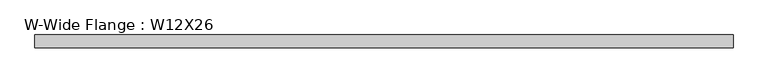
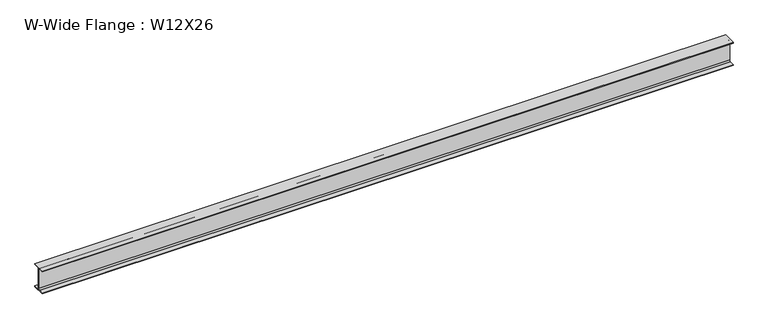
"""IFC4 building model written with IfcOpenShell, lengths in millimetres: beam geometry, W-Wide Flange : W12X26."""

from ifc_helpers import new_model, si_unit, point, frame, frame_2d, origin, place, context, project, spatial, polyline, circle_curve, trimmed, segment, composite_curve, outline, extrude, source, transform, mapped, element, save


def w_wide_flange_w12x26_21dbd052(model_context):
    return source(origin(), model_context, "Body", "SweptSolid", [
        extrude(outline(composite_curve([segment(polyline([(82.4011719, -145.5539063), (82.4011719, -155.178125), (-82.4011719, -155.178125), (-82.4011719, -145.5539063), (-20.2902344, -145.5539063)]), True, "CONTINUOUS"), segment(trimmed(circle_curve(frame_2d((-20.2902344, -128.190625)), 17.3632812), [point((-20.2902344, -145.5539063))], [point((-2.9269531, -128.190625))], True, "CARTESIAN"), True, "CONTINUOUS"), segment(polyline([(-2.9269531, -128.190625), (-2.9269531, 128.190625)]), True, "CONTINUOUS"), segment(trimmed(circle_curve(frame_2d((-20.2902344, 128.190625)), 17.3632812), [point((-2.9269531, 128.190625))], [point((-20.2902344, 145.5539062))], True, "CARTESIAN"), True, "CONTINUOUS"), segment(polyline([(-20.2902344, 145.5539062), (-82.4011719, 145.5539062), (-82.4011719, 155.178125), (82.4011719, 155.178125), (82.4011719, 145.5539062), (20.2902344, 145.5539062)]), True, "CONTINUOUS"), segment(trimmed(circle_curve(frame_2d((20.2902344, 128.190625)), 17.3632812), [point((20.2902344, 145.5539062))], [point((2.9269531, 128.190625))], True, "CARTESIAN"), True, "CONTINUOUS"), segment(polyline([(2.9269531, 128.190625), (2.9269531, -128.190625)]), True, "CONTINUOUS"), segment(trimmed(circle_curve(frame_2d((20.2902344, -128.190625)), 17.3632812), [point((2.9269531, -128.190625))], [point((20.2902344, -145.5539063))], True, "CARTESIAN"), True, "CONTINUOUS"), segment(polyline([(20.2902344, -145.5539063), (82.4011719, -145.5539063)]), True, "CONTINUOUS")], self_intersect=False)), frame((-3657.6, 0.0, 0.0), z_axis=(1.0, 0.0, 0.0), x_axis=(0.0, 1.0, 0.0)), (0.0, 0.0, 1.0), 8839.2),
    ])


if __name__ == "__main__":
    model = new_model("IFC4")
    model_context = context("Model", 3, world=origin())
    ifc_project = project(units=[si_unit("LENGTHUNIT", "METRE", prefix="MILLI")], contexts=[model_context])
    site = spatial("IfcSite", under=ifc_project)
    building = spatial("IfcBuilding", under=site)
    placement = place(None, origin())
    w_wide_flange_w12x26_shape = w_wide_flange_w12x26_21dbd052(model_context)
    element("IfcBeam", 1, ObjectType="W-Wide Flange : W12X26", at=placement, inside=building, context=model_context, shape_type="MappedRepresentation", body=[
        mapped(w_wide_flange_w12x26_shape, transform((0.0, 0.0, 0.0), x_axis=(1.0, 0.0, 0.0), y_axis=(0.0, 1.0, 0.0), z_axis=(0.0, 0.0, 1.0))),
    ])
    save(model, "model.ifc")

# Revit data of these elements
# Type "W-Wide Flange : W12X26"
#   Assembly Code = "B10"
#   W = 26
#   Length [instance default] = 5' - 0"
#   bf = 0' - 6 125/256"
#   d = 1' - 0 7/32"
#   k = 0' - 1 1/16"
#   k2 = 0' - 0 175/256"
#   tf = 0' - 0 97/256"
#   tw = 0' - 0 59/256"
#   A = 0.053125 SF
#   Structural Material [instance default] = none
